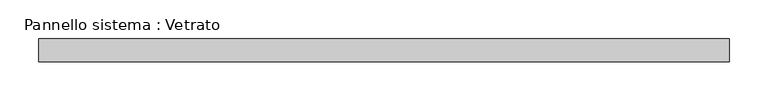
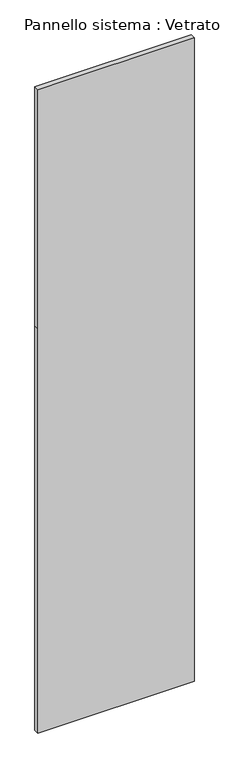
"""IFC4 building model written with IfcOpenShell, lengths in millimetres: plate geometry, Pannello sistema : Vetrato."""

import ifcopenshell
import ifcopenshell.guid

model = None  # the IFC model being written
_history = None  # IfcOwnerHistory: only IFC2X3 demands one
_inside = {}  # id of a spatial element -> (the spatial element, [elements in it])
_under = {}  # id of a project, library or spatial element -> (it, [spatial elements below it])
_declared = {}  # id of a project -> (the project, [libraries it declares])
_typed = {}  # id of a type object -> (the type object, [elements of that type])
_made_of = {}  # id of a material, layer set ... -> (it, [elements and type objects made of it])


def new_model(schema):
    """Start an empty IFC model of exactly this schema.

    Asked for "IFC4X3", IfcOpenShell would pick the latest addendum, in which some entities
    have other attributes; the version numbers below select the first issue.
    IFC2X3 requires an IfcOwnerHistory on every rooted entity: one is made here for all.
    """
    global model, _history
    if schema == "IFC4X3":
        model = ifcopenshell.file(schema_version=(4, 3, 0, 0))
    else:
        model = ifcopenshell.file(schema=schema)
    _inside.clear()
    _under.clear()
    _declared.clear()
    _typed.clear()
    _made_of.clear()
    _history = None
    if model.schema == "IFC2X3":
        org = make("IfcOrganization", Name="unknown")
        user = make(
            "IfcPersonAndOrganization",
            ThePerson=make("IfcPerson", FamilyName="unknown"),
            TheOrganization=org,
        )
        app = make(
            "IfcApplication",
            ApplicationDeveloper=org,
            Version="unknown",
            ApplicationFullName="unknown",
            ApplicationIdentifier="unknown",
        )
        _history = make(
            "IfcOwnerHistory",
            OwningUser=user,
            OwningApplication=app,
            ChangeAction="ADDED",
            CreationDate=0,
        )
    return model


def make(cls, **values):
    """One entity of the class cls with the attributes given. An attribute that is None is left unset."""
    return model.create_entity(
        cls, **{name: value for name, value in values.items() if value is not None}
    )


def rooted(cls, **values):
    """An entity with a GlobalId (a new one), such as an element, a storey or a relation."""
    return make(cls, GlobalId=ifcopenshell.guid.new(), OwnerHistory=_history, **values)


def si_unit(unit_type, name, prefix=None):
    """IfcSIUnit, for example si_unit("LENGTHUNIT", "METRE", prefix="MILLI")."""
    return make("IfcSIUnit", UnitType=unit_type, Prefix=prefix, Name=name)


def assignment(units):
    """IfcUnitAssignment: the units of a project."""
    return None if units is None else make("IfcUnitAssignment", Units=units)


def point(xyz):
    """IfcCartesianPoint."""
    return None if xyz is None else make("IfcCartesianPoint", Coordinates=xyz)


def direction(xyz):
    """IfcDirection."""
    return None if xyz is None else make("IfcDirection", DirectionRatios=xyz)


def frame(location, z_axis=None, x_axis=None):
    """IfcAxis2Placement3D, a coordinate frame: its origin and axes. An axis left out is left unset."""
    return make(
        "IfcAxis2Placement3D",
        Location=point(location),
        Axis=direction(z_axis),
        RefDirection=direction(x_axis),
    )


def origin():
    """The frame at (0, 0, 0) with its axes left unset."""
    return frame((0.0, 0.0, 0.0))


def place(relative_to, where):
    """IfcLocalPlacement: puts the frame where relative to a parent placement (None: the world)."""
    return make(
        "IfcLocalPlacement", PlacementRelTo=relative_to, RelativePlacement=where
    )


def context(
    kind, dimensions, precision=None, world=None, true_north=None, identifier=None
):
    """IfcGeometricRepresentationContext, for example the 3D "Model" context."""
    return make(
        "IfcGeometricRepresentationContext",
        ContextIdentifier=identifier,
        ContextType=kind,
        CoordinateSpaceDimension=dimensions,
        Precision=precision,
        WorldCoordinateSystem=world,
        TrueNorth=true_north,
    )


def project(units=None, contexts=None):
    """IfcProject with its units and contexts."""
    return rooted(
        "IfcProject",
        Name="project",
        RepresentationContexts=contexts,
        UnitsInContext=assignment(units),
    )


def spatial(cls, under=None, at=None, **own):
    """A site, building, storey or space (cls), placed at a placement, below another one or the project."""
    s = rooted(cls, ObjectPlacement=at, **own)
    if under is not None:
        _under.setdefault(under.id(), (under, []))[1].append(s)
    return s


def polyline(points):
    """IfcPolyline through the points."""
    return make("IfcPolyline", Points=[point(p) for p in points])


def outline(outer, holes=None, kind="AREA"):
    """IfcArbitraryClosedProfileDef: a profile drawn as a closed curve; with holes, ...WithVoids."""
    if holes is None:
        return make("IfcArbitraryClosedProfileDef", ProfileType=kind, OuterCurve=outer)
    return make(
        "IfcArbitraryProfileDefWithVoids",
        ProfileType=kind,
        OuterCurve=outer,
        InnerCurves=holes,
    )


def extrude(swept, where, along, depth):
    """IfcExtrudedAreaSolid: the profile swept, set in the frame where, extruded along a direction by depth."""
    return make(
        "IfcExtrudedAreaSolid",
        SweptArea=swept,
        Position=where,
        ExtrudedDirection=direction(along),
        Depth=depth,
    )


def shape(context_of_items, identifier, shape_type, items):
    """IfcShapeRepresentation: the items that make up one representation, for example the "Body"."""
    return make(
        "IfcShapeRepresentation",
        ContextOfItems=context_of_items,
        RepresentationIdentifier=identifier,
        RepresentationType=shape_type,
        Items=items,
    )


def source(mapping_origin, context_of_items, identifier, shape_type, items):
    """IfcRepresentationMap: a shape defined once, which mapped items show again and again."""
    return make(
        "IfcRepresentationMap",
        MappingOrigin=mapping_origin,
        MappedRepresentation=shape(context_of_items, identifier, shape_type, items),
    )


def transform(
    local_origin,
    x_axis=None,
    y_axis=None,
    z_axis=None,
    scale=None,
    scale2=None,
    scale3=None,
    uniform=True,
):
    """IfcCartesianTransformationOperator3D, or its non-uniform kind. x_axis, y_axis, z_axis: its Axis1, 2, 3."""
    if uniform:
        return make(
            "IfcCartesianTransformationOperator3D",
            Axis1=direction(x_axis),
            Axis2=direction(y_axis),
            LocalOrigin=point(local_origin),
            Scale=scale,
            Axis3=direction(z_axis),
        )
    return make(
        "IfcCartesianTransformationOperator3DnonUniform",
        Axis1=direction(x_axis),
        Axis2=direction(y_axis),
        LocalOrigin=point(local_origin),
        Scale=scale,
        Axis3=direction(z_axis),
        Scale2=scale2,
        Scale3=scale3,
    )


def mapped(mapping_source, mapping_target):
    """IfcMappedItem: shows the shape of a source again, moved by a transform."""
    return make(
        "IfcMappedItem", MappingSource=mapping_source, MappingTarget=mapping_target
    )


def made_of(thing, what):
    """Note that an element or type object is made of a material, layer set ...; save() writes the relation."""
    if what is not None:
        _made_of.setdefault(what.id(), (what, []))[1].append(thing)
    return thing


def element(
    cls,
    number,
    at=None,
    inside=None,
    cuts=None,
    type_object=None,
    material=None,
    context=None,
    identifier="Body",
    shape_type=None,
    held_by="IfcProductDefinitionShape",
    body=None,
    shapes=None,
    **own,
):
    """One element of the class cls, such as IfcWall. Its Tag is "e" and its number.

    at: its placement. inside: the storey or other place that contains it. cuts: it is an
    opening in that element (IfcRelVoidsElement). A single representation is given by context,
    identifier, shape_type and body (its items); several are given by shapes. held_by: the class
    of the entity that holds the representations. save() writes the other relations.
    """
    e = rooted(cls, Tag="e%d" % number, ObjectPlacement=at, **own)
    if body is not None:
        shapes = [shape(context, identifier, shape_type, body)]
    if shapes is not None:
        e.Representation = make(held_by, Representations=shapes)
    if inside is not None:
        _inside.setdefault(inside.id(), (inside, []))[1].append(e)
    if cuts is not None:
        rooted(
            "IfcRelVoidsElement", RelatingBuildingElement=cuts, RelatedOpeningElement=e
        )
    if type_object is not None:
        _typed.setdefault(type_object.id(), (type_object, []))[1].append(e)
    return made_of(e, material)


def aggregate(whole, parts):
    """IfcRelAggregates: a whole, such as a stair, and the parts it consists of."""
    return rooted("IfcRelAggregates", RelatingObject=whole, RelatedObjects=parts)


def save(model, path):
    """Write the relations noted so far, then the file.

    IfcRelAggregates (storeys below a building ...), IfcRelContainedInSpatialStructure (elements
    in a storey), IfcRelDefinesByType, IfcRelAssociatesMaterial and IfcRelDeclares: one each for
    every whole, place, type object, material and project.
    """
    for whole, parts in _under.values():
        aggregate(whole, parts)
    for where, things in _inside.values():
        rooted(
            "IfcRelContainedInSpatialStructure",
            RelatedElements=things,
            RelatingStructure=where,
        )
    for kind, things in _typed.values():
        rooted("IfcRelDefinesByType", RelatedObjects=things, RelatingType=kind)
    for what, things in _made_of.values():
        rooted("IfcRelAssociatesMaterial", RelatedObjects=things, RelatingMaterial=what)
    for by, libraries in _declared.values():
        rooted("IfcRelDeclares", RelatingContext=by, RelatedDefinitions=libraries)
    model.write(path)


def pannello_sistema_vetrato_00c806ab(model_context):
    return source(origin(), model_context, "Body", "SweptSolid", [
        extrude(outline(polyline([(0.0, -447.5), (0.0, 447.5), (2450.0, 447.5), (3900.0, 447.5), (3900.0, -447.5), (2450.0, -447.5), (0.0, -447.5)])), frame((0.0, -15.0, 0.0), z_axis=(0.0, 1.0, 0.0), x_axis=(0.0, 0.0, 1.0)), (0.0, 0.0, 1.0), 30.0),
    ])


if __name__ == "__main__":
    model = new_model("IFC4")
    model_context = context("Model", 3, world=origin())
    ifc_project = project(units=[si_unit("LENGTHUNIT", "METRE", prefix="MILLI")], contexts=[model_context])
    site = spatial("IfcSite", under=ifc_project)
    building = spatial("IfcBuilding", under=site)
    placement = place(None, origin())
    pannello_sistema_vetrato_shape = pannello_sistema_vetrato_00c806ab(model_context)
    element("IfcPlate", 1, ObjectType="Pannello sistema : Vetrato", at=placement, inside=building, context=model_context, shape_type="MappedRepresentation", body=[
        mapped(pannello_sistema_vetrato_shape, transform((0.0, 0.0, 0.0), x_axis=(1.0, 0.0, 0.0), y_axis=(0.0, 1.0, 0.0), z_axis=(0.0, 0.0, 1.0))),
    ])
    save(model, "model.ifc")

# Revit data of these elements
# Project information
#   Data di consegna del progetto = "Data"
#   Stato del progetto = "Stato"
#   Nome del cliente = "Proprietario"
#   Nome del progetto = "Nome"
#   Numero del progetto = "0001"
# Type "Pannello sistema : Vetrato"
#   Construction Type Id = "GSP4R"
#   Analytic Construction = "Vetrata singola Pilkington 1/8 in"
#   Visual Light Transmittance = 0.9
#   Solar Heat Gain Coefficient = 0.86
#   Heat Transfer Coefficient (U) = 6.7069 W/(m²·K)
# Element 1 (IfcPlate, "Pannello sistema : Vetrato")
#   Materials on its faces: "Default - Vetro"
# Materials
#   "Default - Vetro": class "Vetro", colour RGB 208 208 208, transparency 0.7, Cost = 0
